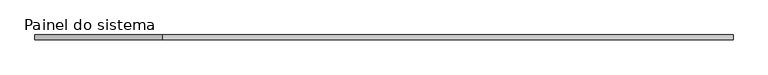
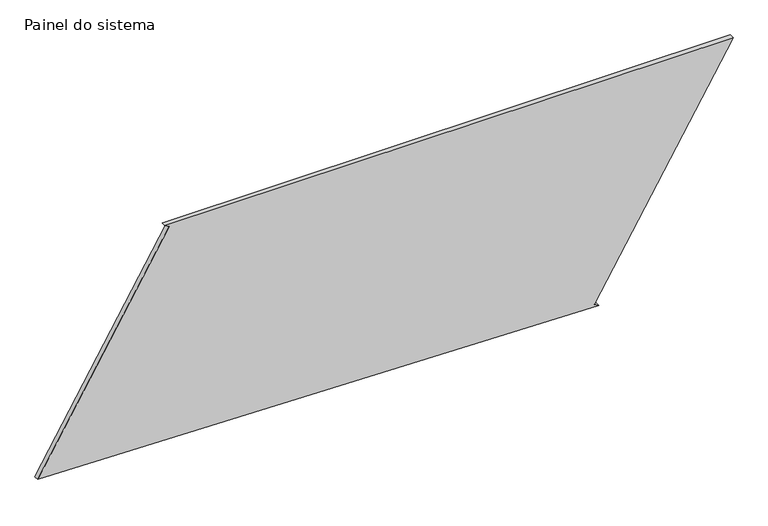
"""IFC4 building model written with IfcOpenShell, lengths in millimetres: plate geometry, Painel do sistema : Envidraçado."""

from ifc_helpers import new_model, si_unit, frame, origin, place, context, project, spatial, polyline, outline, extrude, source, transform, mapped, element, save


def painel_do_sistema_1a0cbb23(model_context):
    return source(origin(), model_context, "Body", "SweptSolid", [
        extrude(outline(polyline([(0.0, 1111.4966135), (12.7505939, 1089.9926056), (1231.7149264, 1812.7657437), (1231.7149264, -1149.0413703), (1218.9643324, -1127.5373624), (63.3196186, -1812.7657437), (0.0, 1111.4966135)])), frame((0.0, 24.5, 0.0), z_axis=(0.0, 1.0, 0.0), x_axis=(0.0, 0.0, 1.0)), (0.0, 0.0, 1.0), 25.0),
    ])


if __name__ == "__main__":
    model = new_model("IFC4")
    model_context = context("Model", 3, world=origin())
    ifc_project = project(units=[si_unit("LENGTHUNIT", "METRE", prefix="MILLI")], contexts=[model_context])
    site = spatial("IfcSite", under=ifc_project)
    building = spatial("IfcBuilding", under=site)
    placement = place(None, origin())
    painel_do_sistema_shape = painel_do_sistema_1a0cbb23(model_context)
    element("IfcPlate", 1, ObjectType="Painel do sistema : Envidraçado", at=placement, inside=building, context=model_context, shape_type="MappedRepresentation", body=[
        mapped(painel_do_sistema_shape, transform((0.0, 0.0, 0.0), x_axis=(1.0, 0.0, 0.0), y_axis=(0.0, 1.0, 0.0), z_axis=(0.0, 0.0, 1.0))),
    ])
    save(model, "model.ifc")

# Revit data of these elements
# Type "Painel do sistema : Envidraçado"
#   Construction Type Id = "GSP4R"
#   Analytic Construction = "Vidraça única Pilkington 1/8 pol"
#   Visual Light Transmittance = 0.9
#   Solar Heat Gain Coefficient = 0.86
#   Heat Transfer Coefficient (U) = 6.7069 W/(m²·K)
# Element 1 (IfcPlate, "Painel do sistema : Envidraçado")
#   Materials on its faces: "Vidro"
# Materials
#   "Vidro": class "Vidro", colour RGB 0 128 192, transparency 0.9, Description = "Vidro de sílica", Cost = 0
